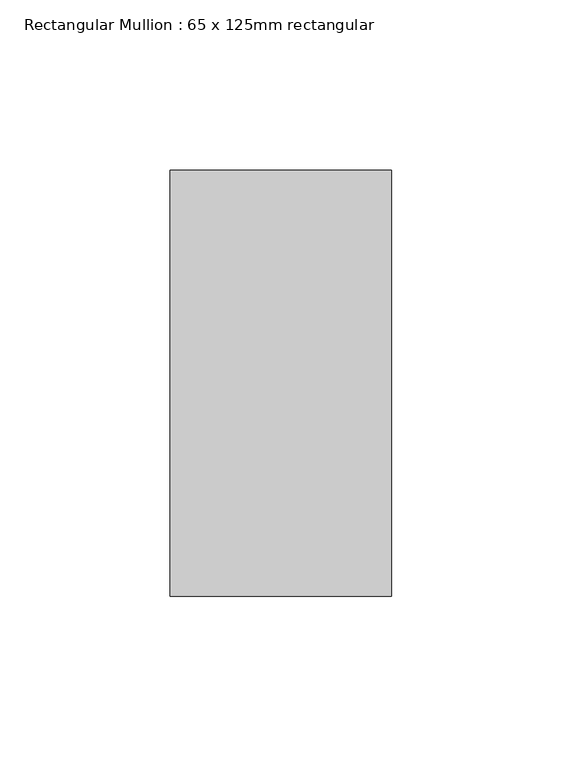
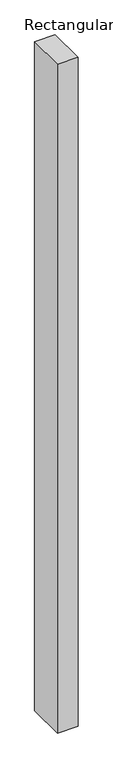
"""IFC4 building model written with IfcOpenShell, lengths in millimetres: member geometry, Rectangular Mullion : 65 x 125mm rectangular."""

from ifc_helpers import new_model, si_unit, frame, origin, place, context, project, spatial, polyline, outline, extrude, source, transform, mapped, element, save


def rectangular_mullion_65_x_125mm_rectangular_245190dc(model_context):
    return source(origin(), model_context, "Body", "SweptSolid", [
        extrude(outline(polyline([(0.0, 62.5), (0.0, -62.5), (-65.0, -62.5), (-65.0, 62.5), (0.0, 62.5)])), frame((0.0, 0.0, -2244.830414), z_axis=(0.0, 0.0, 1.0), x_axis=(1.0, 0.0, 0.0)), (0.0, 0.0, 1.0), 2244.830414),
    ])


if __name__ == "__main__":
    model = new_model("IFC4")
    model_context = context("Model", 3, world=origin())
    ifc_project = project(units=[si_unit("LENGTHUNIT", "METRE", prefix="MILLI")], contexts=[model_context])
    site = spatial("IfcSite", under=ifc_project)
    building = spatial("IfcBuilding", under=site)
    placement = place(None, origin())
    rectangular_mullion_65_x_125mm_rectangular_shape = rectangular_mullion_65_x_125mm_rectangular_245190dc(model_context)
    element("IfcMember", 1, ObjectType="Rectangular Mullion : 65 x 125mm rectangular", at=placement, inside=building, context=model_context, shape_type="MappedRepresentation", body=[
        mapped(rectangular_mullion_65_x_125mm_rectangular_shape, transform((0.0, 0.0, 0.0), x_axis=(1.0, 0.0, 0.0), y_axis=(0.0, 1.0, 0.0), z_axis=(0.0, 0.0, 1.0))),
    ])
    save(model, "model.ifc")

# Revit data of these elements
# Type "Rectangular Mullion : 65 x 125mm rectangular"
#   built-in parameter 1007304 = 0.410105 (stored number, unit not read)
#   built-in parameter 1007301 = 0.106627 (stored number, unit not read)
#   built-in parameter 1007300 = 0.106627 (stored number, unit not read)
# Element 1 (IfcMember, "Rectangular Mullion : 65 x 125mm rectangular")
#   Materials on its faces: "Aluminum"
# Materials
#   "Aluminum": class "Metal", colour RGB 244 245 246, transparency 0, Description = "Aluminum 6061", Cost = 0
